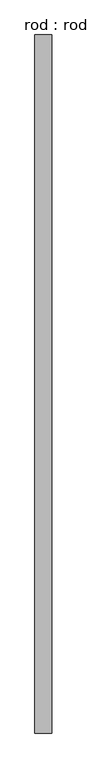
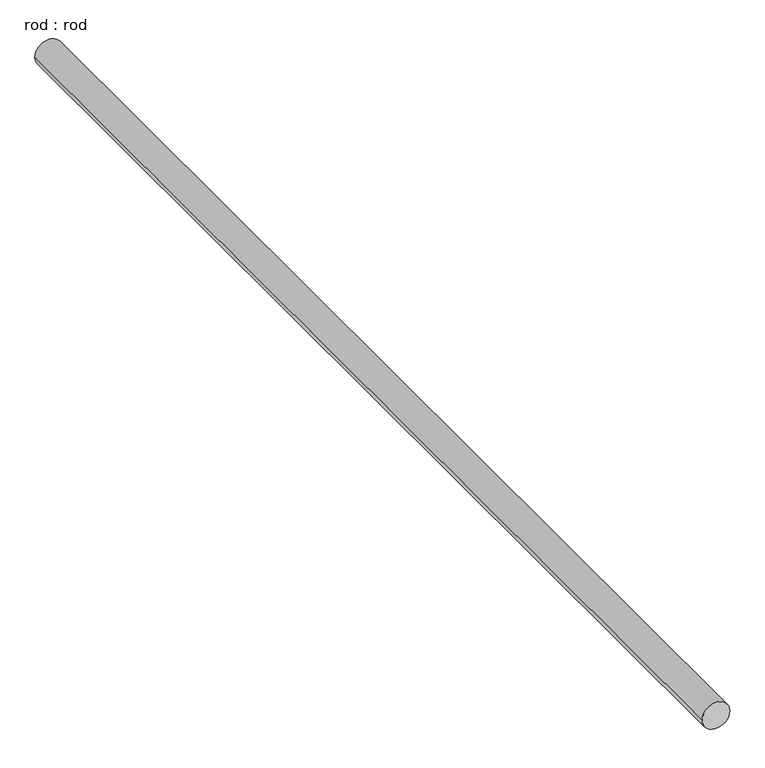
"""IFC4 building model written with IfcOpenShell, lengths in millimetres: proxy geometry, rod : rod."""

from ifc_helpers import new_model, si_unit, point, frame, frame_2d, origin, place, context, project, spatial, circle_curve, trimmed, segment, composite_curve, outline, extrude, source, transform, mapped, element, save


def rod_rod_348e3640(model_context):
    return source(origin(), model_context, "Body", "SweptSolid", [
        extrude(outline(composite_curve([segment(trimmed(circle_curve(frame_2d((0.0108462, 0.0)), 200.0), [point((0.0108462, 200.0))], [point((0.0108462, -200.0))], False, "CARTESIAN"), True, "CONTINUOUS"), segment(trimmed(circle_curve(frame_2d((0.0108462, 0.0)), 200.0), [point((0.0108462, -200.0))], [point((0.0108462, 200.0))], False, "CARTESIAN"), True, "CONTINUOUS")], self_intersect=False)), frame((0.0, -4264.4142418, 0.0), z_axis=(0.0, 1.0, 0.0), x_axis=(0.0, 0.0, 1.0)), (0.0, 0.0, 1.0), 16714.2857143),
    ])


if __name__ == "__main__":
    model = new_model("IFC4")
    model_context = context("Model", 3, world=origin())
    ifc_project = project(units=[si_unit("LENGTHUNIT", "METRE", prefix="MILLI")], contexts=[model_context])
    site = spatial("IfcSite", under=ifc_project)
    building = spatial("IfcBuilding", under=site)
    placement = place(None, origin())
    rod_rod_shape = rod_rod_348e3640(model_context)
    element("IfcBuildingElementProxy", 1, Name="rod : rod", ObjectType="rod : rod", at=placement, inside=building, context=model_context, shape_type="MappedRepresentation", body=[
        mapped(rod_rod_shape, transform((0.0, 0.0, 0.0), x_axis=(1.0, 0.0, 0.0), y_axis=(0.0, 1.0, 0.0), z_axis=(0.0, 0.0, 1.0))),
    ])
    save(model, "model.ifc")

# Revit data of these elements
# Type "rod : rod"
#   Default Elevation = 0
